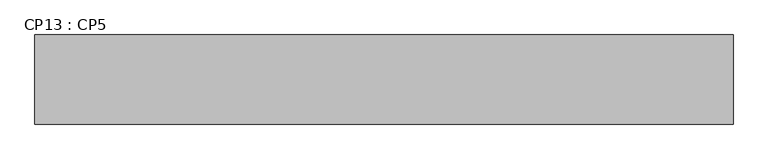
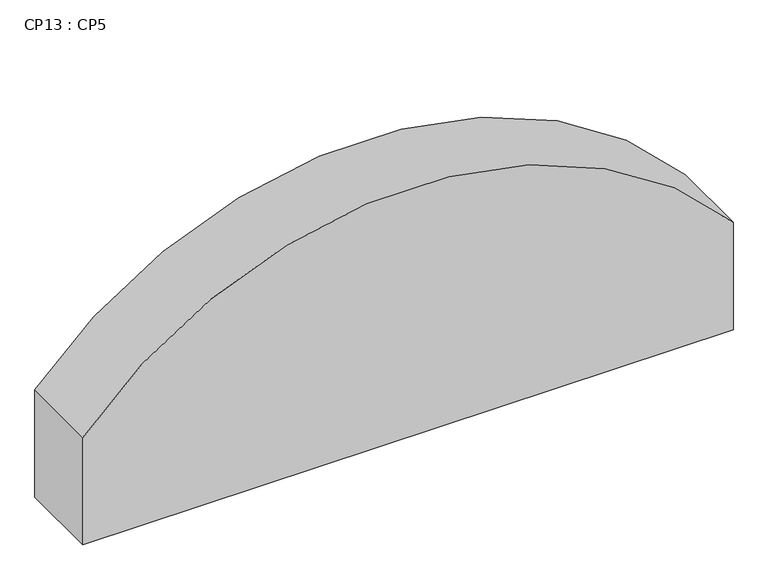
"""IFC4 building model written with IfcOpenShell, lengths in millimetres: beam geometry, CP13 : CP5."""

import ifcopenshell
import ifcopenshell.guid

model = None  # the IFC model being written
_history = None  # IfcOwnerHistory: only IFC2X3 demands one
_inside = {}  # id of a spatial element -> (the spatial element, [elements in it])
_under = {}  # id of a project, library or spatial element -> (it, [spatial elements below it])
_declared = {}  # id of a project -> (the project, [libraries it declares])
_typed = {}  # id of a type object -> (the type object, [elements of that type])
_made_of = {}  # id of a material, layer set ... -> (it, [elements and type objects made of it])


def new_model(schema):
    """Start an empty IFC model of exactly this schema.

    Asked for "IFC4X3", IfcOpenShell would pick the latest addendum, in which some entities
    have other attributes; the version numbers below select the first issue.
    IFC2X3 requires an IfcOwnerHistory on every rooted entity: one is made here for all.
    """
    global model, _history
    if schema == "IFC4X3":
        model = ifcopenshell.file(schema_version=(4, 3, 0, 0))
    else:
        model = ifcopenshell.file(schema=schema)
    _inside.clear()
    _under.clear()
    _declared.clear()
    _typed.clear()
    _made_of.clear()
    _history = None
    if model.schema == "IFC2X3":
        org = make("IfcOrganization", Name="unknown")
        user = make(
            "IfcPersonAndOrganization",
            ThePerson=make("IfcPerson", FamilyName="unknown"),
            TheOrganization=org,
        )
        app = make(
            "IfcApplication",
            ApplicationDeveloper=org,
            Version="unknown",
            ApplicationFullName="unknown",
            ApplicationIdentifier="unknown",
        )
        _history = make(
            "IfcOwnerHistory",
            OwningUser=user,
            OwningApplication=app,
            ChangeAction="ADDED",
            CreationDate=0,
        )
    return model


def make(cls, **values):
    """One entity of the class cls with the attributes given. An attribute that is None is left unset."""
    return model.create_entity(
        cls, **{name: value for name, value in values.items() if value is not None}
    )


def rooted(cls, **values):
    """An entity with a GlobalId (a new one), such as an element, a storey or a relation."""
    return make(cls, GlobalId=ifcopenshell.guid.new(), OwnerHistory=_history, **values)


def si_unit(unit_type, name, prefix=None):
    """IfcSIUnit, for example si_unit("LENGTHUNIT", "METRE", prefix="MILLI")."""
    return make("IfcSIUnit", UnitType=unit_type, Prefix=prefix, Name=name)


def assignment(units):
    """IfcUnitAssignment: the units of a project."""
    return None if units is None else make("IfcUnitAssignment", Units=units)


def point(xyz):
    """IfcCartesianPoint."""
    return None if xyz is None else make("IfcCartesianPoint", Coordinates=xyz)


def direction(xyz):
    """IfcDirection."""
    return None if xyz is None else make("IfcDirection", DirectionRatios=xyz)


def frame(location, z_axis=None, x_axis=None):
    """IfcAxis2Placement3D, a coordinate frame: its origin and axes. An axis left out is left unset."""
    return make(
        "IfcAxis2Placement3D",
        Location=point(location),
        Axis=direction(z_axis),
        RefDirection=direction(x_axis),
    )


def origin():
    """The frame at (0, 0, 0) with its axes left unset."""
    return frame((0.0, 0.0, 0.0))


def place(relative_to, where):
    """IfcLocalPlacement: puts the frame where relative to a parent placement (None: the world)."""
    return make(
        "IfcLocalPlacement", PlacementRelTo=relative_to, RelativePlacement=where
    )


def context(
    kind, dimensions, precision=None, world=None, true_north=None, identifier=None
):
    """IfcGeometricRepresentationContext, for example the 3D "Model" context."""
    return make(
        "IfcGeometricRepresentationContext",
        ContextIdentifier=identifier,
        ContextType=kind,
        CoordinateSpaceDimension=dimensions,
        Precision=precision,
        WorldCoordinateSystem=world,
        TrueNorth=true_north,
    )


def project(units=None, contexts=None):
    """IfcProject with its units and contexts."""
    return rooted(
        "IfcProject",
        Name="project",
        RepresentationContexts=contexts,
        UnitsInContext=assignment(units),
    )


def spatial(cls, under=None, at=None, **own):
    """A site, building, storey or space (cls), placed at a placement, below another one or the project."""
    s = rooted(cls, ObjectPlacement=at, **own)
    if under is not None:
        _under.setdefault(under.id(), (under, []))[1].append(s)
    return s


def circle_curve(where, radius):
    """IfcCircle in the frame where."""
    return make("IfcCircle", Position=where, Radius=radius)


def shape(context_of_items, identifier, shape_type, items):
    """IfcShapeRepresentation: the items that make up one representation, for example the "Body"."""
    return make(
        "IfcShapeRepresentation",
        ContextOfItems=context_of_items,
        RepresentationIdentifier=identifier,
        RepresentationType=shape_type,
        Items=items,
    )


def source(mapping_origin, context_of_items, identifier, shape_type, items):
    """IfcRepresentationMap: a shape defined once, which mapped items show again and again."""
    return make(
        "IfcRepresentationMap",
        MappingOrigin=mapping_origin,
        MappedRepresentation=shape(context_of_items, identifier, shape_type, items),
    )


def transform(
    local_origin,
    x_axis=None,
    y_axis=None,
    z_axis=None,
    scale=None,
    scale2=None,
    scale3=None,
    uniform=True,
):
    """IfcCartesianTransformationOperator3D, or its non-uniform kind. x_axis, y_axis, z_axis: its Axis1, 2, 3."""
    if uniform:
        return make(
            "IfcCartesianTransformationOperator3D",
            Axis1=direction(x_axis),
            Axis2=direction(y_axis),
            LocalOrigin=point(local_origin),
            Scale=scale,
            Axis3=direction(z_axis),
        )
    return make(
        "IfcCartesianTransformationOperator3DnonUniform",
        Axis1=direction(x_axis),
        Axis2=direction(y_axis),
        LocalOrigin=point(local_origin),
        Scale=scale,
        Axis3=direction(z_axis),
        Scale2=scale2,
        Scale3=scale3,
    )


def mapped(mapping_source, mapping_target):
    """IfcMappedItem: shows the shape of a source again, moved by a transform."""
    return make(
        "IfcMappedItem", MappingSource=mapping_source, MappingTarget=mapping_target
    )


def made_of(thing, what):
    """Note that an element or type object is made of a material, layer set ...; save() writes the relation."""
    if what is not None:
        _made_of.setdefault(what.id(), (what, []))[1].append(thing)
    return thing


def element(
    cls,
    number,
    at=None,
    inside=None,
    cuts=None,
    type_object=None,
    material=None,
    context=None,
    identifier="Body",
    shape_type=None,
    held_by="IfcProductDefinitionShape",
    body=None,
    shapes=None,
    **own,
):
    """One element of the class cls, such as IfcWall. Its Tag is "e" and its number.

    at: its placement. inside: the storey or other place that contains it. cuts: it is an
    opening in that element (IfcRelVoidsElement). A single representation is given by context,
    identifier, shape_type and body (its items); several are given by shapes. held_by: the class
    of the entity that holds the representations. save() writes the other relations.
    """
    e = rooted(cls, Tag="e%d" % number, ObjectPlacement=at, **own)
    if body is not None:
        shapes = [shape(context, identifier, shape_type, body)]
    if shapes is not None:
        e.Representation = make(held_by, Representations=shapes)
    if inside is not None:
        _inside.setdefault(inside.id(), (inside, []))[1].append(e)
    if cuts is not None:
        rooted(
            "IfcRelVoidsElement", RelatingBuildingElement=cuts, RelatedOpeningElement=e
        )
    if type_object is not None:
        _typed.setdefault(type_object.id(), (type_object, []))[1].append(e)
    return made_of(e, material)


def aggregate(whole, parts):
    """IfcRelAggregates: a whole, such as a stair, and the parts it consists of."""
    return rooted("IfcRelAggregates", RelatingObject=whole, RelatedObjects=parts)


def save(model, path):
    """Write the relations noted so far, then the file.

    IfcRelAggregates (storeys below a building ...), IfcRelContainedInSpatialStructure (elements
    in a storey), IfcRelDefinesByType, IfcRelAssociatesMaterial and IfcRelDeclares: one each for
    every whole, place, type object, material and project.
    """
    for whole, parts in _under.values():
        aggregate(whole, parts)
    for where, things in _inside.values():
        rooted(
            "IfcRelContainedInSpatialStructure",
            RelatedElements=things,
            RelatingStructure=where,
        )
    for kind, things in _typed.values():
        rooted("IfcRelDefinesByType", RelatedObjects=things, RelatingType=kind)
    for what, things in _made_of.values():
        rooted("IfcRelAssociatesMaterial", RelatedObjects=things, RelatingMaterial=what)
    for by, libraries in _declared.values():
        rooted("IfcRelDeclares", RelatingContext=by, RelatedDefinitions=libraries)
    model.write(path)


def plane_surface(at):
    """IfcPlane: the flat surface through the origin of the frame at, square to its z axis."""
    return make("IfcPlane", Position=at)


def cylinder_surface(at, radius):
    """IfcCylindricalSurface: all points at the distance radius from the z axis of the frame at."""
    return make("IfcCylindricalSurface", Position=at, Radius=radius)


def advanced_brep(points, edges, surfaces, faces):
    """IfcAdvancedBrep: a solid bounded by faces that lie on surfaces and meet in shared edges.

    An edge is (start, end): straight between two places in points (the first is 0);
    or (start, end, curve); or (start, end, curve, False) where it runs against its curve.
    A face is (place in surfaces, loops), or (place, loops, False) where it looks against
    its surface's normal. A loop lists edges by number (the first is 1), with a minus sign
    where the edge is run from its end to its start. The first loop is the outer one.
    """
    corners = [point(p) for p in points]
    vertices = [make("IfcVertexPoint", VertexGeometry=c) for c in corners]
    made = []
    for start, end, *more in edges:
        made.append(
            make(
                "IfcEdgeCurve",
                EdgeStart=vertices[start],
                EdgeEnd=vertices[end],
                EdgeGeometry=more[0] if more else make("IfcPolyline", Points=[corners[start], corners[end]]),
                SameSense=more[1] if len(more) > 1 else True,
            )
        )
    hull = []
    for where, loops, *sense in faces:
        bounds = []
        for j, loop in enumerate(loops):
            ring = [make("IfcOrientedEdge", EdgeElement=made[abs(k) - 1], Orientation=k > 0) for k in loop]
            bounds.append(
                make(
                    "IfcFaceOuterBound" if j == 0 else "IfcFaceBound",
                    Bound=make("IfcEdgeLoop", EdgeList=ring),
                    Orientation=True,
                )
            )
        hull.append(make("IfcAdvancedFace", Bounds=bounds, FaceSurface=surfaces[where], SameSense=sense[0] if sense else True))
    return make("IfcAdvancedBrep", Outer=make("IfcClosedShell", CfsFaces=hull))


def cp13_cp5_5f1e0e1f(model_context):
    return source(origin(), model_context, "Body", "AdvancedBrep", [
        advanced_brep(
        [(25483.2245516, 499.6999991, 14620.0), (30183.2245515, 499.6999991, 14620.0), (30183.2245488, 499.6999991, 13800.0), (25483.2245494, 499.6999991, 13800.0), (30183.2245515, -100.2551788, 14620.0), (25483.2245516, -100.2551788, 14620.0), (25483.2245494, -100.2551788, 13800.0), (30183.2245488, -100.2551788, 13800.0)],
        [
            (0, 1, circle_curve(frame((27833.2245515, 499.6999991, 12608.2612414), z_axis=(0.0, 1.0, 0.0), x_axis=(0.0, 0.0, -1.0)), 3093.4758497)),
            (1, 2),
            (2, 3),
            (3, 0),
            (4, 5, circle_curve(frame((27833.2245515, -100.2551788, 12608.2612414), z_axis=(0.0, -1.0, 0.0), x_axis=(0.0, 0.0, -1.0)), 3093.4758497)),
            (5, 6),
            (6, 7),
            (7, 4),
            (2, 7),
            (6, 3),
            (0, 5),
            (4, 1),
        ],
        [
            plane_surface(frame((27758.2245515, 499.6999991, 9004.7654345), z_axis=(0.0, 1.0, 0.0), x_axis=(-1.0, 0.0, 0.0))),
            plane_surface(frame((27758.2245515, -100.2551788, 9004.7654345), z_axis=(0.0, -1.0, 0.0), x_axis=(1.0, 0.0, 0.0))),
            plane_surface(frame((30333.2245515, 499.6999991, 13800.0), z_axis=(0.0, 0.0, -1.0), x_axis=(0.0, -1.0, 0.0))),
            cylinder_surface(frame((27833.2245515, 20099.7448193, 12608.2612414), z_axis=(0.0, 1.0, 0.0), x_axis=(0.0, 0.0, -1.0)), 3093.4758497),
            plane_surface(frame((30183.2245488, 18587.0448193, 13800.0), z_axis=(1.0, 0.0, 0.0), x_axis=(0.0, -1.0, 0.0))),
            plane_surface(frame((25483.2245494, 18587.0448193, 14620.0), z_axis=(-1.0, 0.0, 0.0), x_axis=(0.0, -1.0, 0.0))),
        ],
        [
            (0, [[1, 2, 3, 4]]),
            (1, [[5, 6, 7, 8]]),
            (2, [[9, -7, 10, -3]]),
            (3, [[-1, 11, -5, 12]]),
            (4, [[-2, -12, -8, -9]]),
            (5, [[-4, -10, -6, -11]]),
        ],
    ),
    ])


if __name__ == "__main__":
    model = new_model("IFC4")
    model_context = context("Model", 3, world=origin())
    ifc_project = project(units=[si_unit("LENGTHUNIT", "METRE", prefix="MILLI")], contexts=[model_context])
    site = spatial("IfcSite", under=ifc_project)
    building = spatial("IfcBuilding", under=site)
    placement = place(None, origin())
    cp13_cp5_shape = cp13_cp5_5f1e0e1f(model_context)
    element("IfcBeam", 1, ObjectType="CP13 : CP5", at=placement, inside=building, context=model_context, shape_type="MappedRepresentation", body=[
        mapped(cp13_cp5_shape, transform((0.0, 0.0, 0.0), x_axis=(1.0, 0.0, 0.0), y_axis=(0.0, 1.0, 0.0), z_axis=(0.0, 0.0, 1.0))),
    ])
    save(model, "model.ifc")
